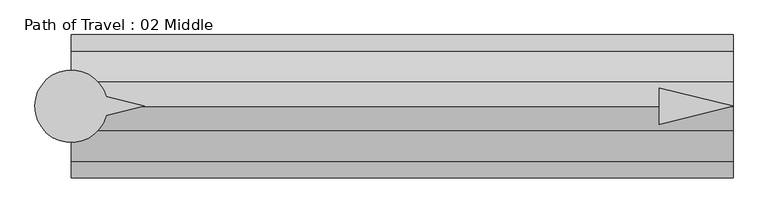
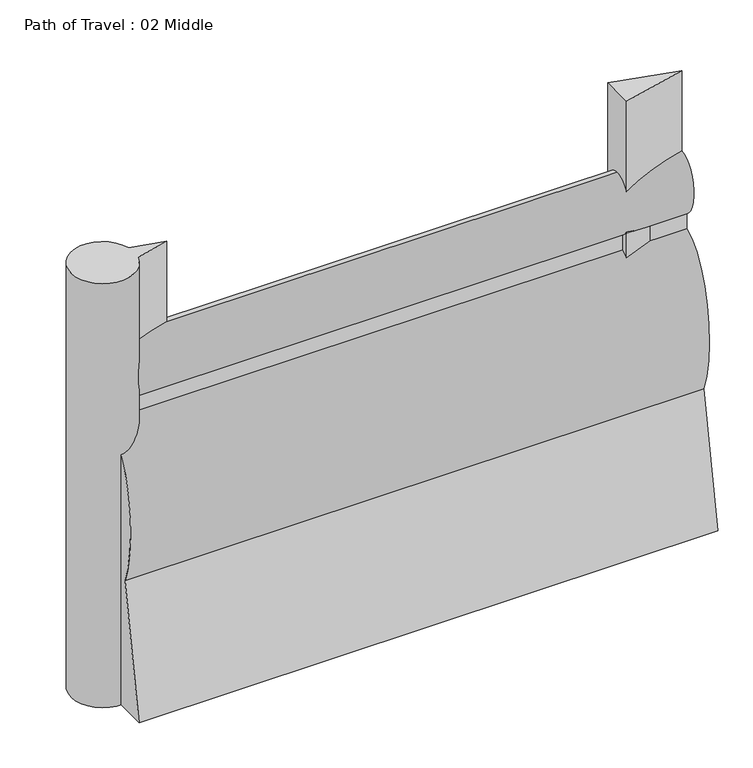
"""IFC4 building model written with IfcOpenShell, lengths in millimetres: proxy geometry, Path of Travel : 02 Middle."""

from ifc_helpers import new_model, si_unit, point, frame, frame_2d, origin, origin_with_axes, place, context, project, spatial, polyline, circle_curve, ellipse_curve, trimmed, segment, composite_curve, outline, extrude, source, transform, mapped, element, save
from ifc_brep_helpers import plane_surface, extruded_surface, advanced_brep


def path_of_travel_02_middle_a2a4b6ed(model_context):
    return source(origin(), model_context, "Body", "SolidModel", [
        advanced_brep(
        [(227.5554837, 0.0, 1727.2), (227.5554837, 42.9018657, 1436.6534209), (227.5554837, 42.9018657, 1363.4763406), (227.5554837, 184.1186263, 643.4144547), (227.5554837, 297.5699544, 0.0), (227.5554837, 145.6574193, 0.0), (227.5554837, 0.0, 584.2), (227.5554837, -145.6574193, 0.0), (227.5554837, -297.5699544, 0.0), (227.5554837, -184.1186263, 643.4144547), (227.5554837, -42.9018657, 1363.4763406), (227.5554837, -42.9018657, 1436.6534209), (2978.9406446, 0.0, 1727.2), (2978.9406446, -42.9018657, 1436.6534209), (2978.9406446, -42.9018657, 1363.4763406), (2978.9406446, -184.1186263, 643.4144547), (2978.9406446, -297.5699544, 0.0), (2978.9406446, -145.6574193, 0.0), (2978.9406446, 0.0, 584.2), (2978.9406446, 145.6574193, 0.0), (2978.9406446, 297.5699544, 0.0), (2978.9406446, 184.1186263, 643.4144547), (2978.9406446, 42.9018657, 1363.4763406), (2978.9406446, 42.9018657, 1436.6534209)],
        [
            (0, 1, ellipse_curve(frame((227.5554837, 0.0, 1574.8), z_axis=(-1.0, 0.0, 0.0), x_axis=(0.0, 0.0, 1.0)), 152.4, 101.6)),
            (1, 2),
            (2, 3, ellipse_curve(frame((227.5554837, 0.0, 914.4), z_axis=(-1.0, 0.0, 0.0), x_axis=(0.0, 0.0, -1.0)), 457.2, 228.6)),
            (3, 4),
            (4, 5),
            (5, 6),
            (6, 7),
            (7, 8),
            (8, 9),
            (9, 10, ellipse_curve(frame((227.5554837, 0.0, 914.4), z_axis=(-1.0, 0.0, 0.0), x_axis=(0.0, 0.0, -1.0)), 457.2, 228.6)),
            (10, 11),
            (11, 0, ellipse_curve(frame((227.5554837, 0.0, 1574.8), z_axis=(-1.0, 0.0, 0.0), x_axis=(0.0, 0.0, 1.0)), 152.4, 101.6)),
            (12, 13, ellipse_curve(frame((2978.9406446, 0.0, 1574.8), z_axis=(1.0, 0.0, 0.0), x_axis=(0.0, 0.0, 1.0)), 152.4, 101.6)),
            (13, 14),
            (14, 15, ellipse_curve(frame((2978.9406446, 0.0, 914.4), z_axis=(1.0, 0.0, 0.0), x_axis=(0.0, 0.0, -1.0)), 457.2, 228.6)),
            (15, 16),
            (16, 17),
            (17, 18),
            (18, 19),
            (19, 20),
            (20, 21),
            (21, 22, ellipse_curve(frame((2978.9406446, 0.0, 914.4), z_axis=(1.0, 0.0, 0.0), x_axis=(0.0, 0.0, -1.0)), 457.2, 228.6)),
            (22, 23),
            (23, 12, ellipse_curve(frame((2978.9406446, 0.0, 1574.8), z_axis=(1.0, 0.0, 0.0), x_axis=(0.0, 0.0, 1.0)), 152.4, 101.6)),
            (0, 12),
            (23, 1),
            (22, 2),
            (21, 3),
            (20, 4),
            (19, 5),
            (18, 6),
            (17, 7),
            (16, 8),
            (15, 9),
            (14, 10),
            (13, 11),
        ],
        [
            plane_surface(frame((227.5554837, 0.0, 0.0), z_axis=(-1.0, 0.0, 0.0), x_axis=(0.0, 0.0, 1.0))),
            plane_surface(frame((2978.9406446, 0.0, 0.0), z_axis=(1.0, 0.0, 0.0), x_axis=(0.0, 0.0, 1.0))),
            extruded_surface(trimmed(ellipse_curve(frame((2978.9406446, 0.0, 1574.8), z_axis=(-1.0, 0.0, 0.0), x_axis=(0.0, 0.0, 1.0)), 152.4, 101.6), [point((2978.9406446, 0.0, 1727.2))], [point((2978.9406446, 42.9018657, 1436.6534209))], True, "CARTESIAN"), (-2751.3851609, 0.0, 0.0), 2751.3851609),
            plane_surface(frame((227.5554837, 42.9018657, 1436.6534209), z_axis=(0.0, 1.0, 0.0), x_axis=(1.0, 0.0, 0.0))),
            extruded_surface(trimmed(ellipse_curve(frame((2978.9406446, 0.0, 914.4), z_axis=(-1.0, 0.0, 0.0), x_axis=(0.0, 0.0, -1.0)), 457.2, 228.6), [point((2978.9406446, 42.9018657, 1363.4763406))], [point((2978.9406446, 184.1186263, 643.4144547))], True, "CARTESIAN"), (-2751.3851609, 0.0, 0.0), 2751.3851609),
            plane_surface(frame((227.5554837, 184.1186263, 643.4144547), z_axis=(0.0, 0.9848077530122078, 0.1736481776669322), x_axis=(1.0, 0.0, 0.0))),
            plane_surface(frame((227.5554837, 297.5699544, 0.0), z_axis=(0.0, 0.0, -1.0), x_axis=(1.0, 0.0, 0.0))),
            plane_surface(frame((227.5554837, 145.6574193, 0.0), z_axis=(0.0, -0.9702957262760199, -0.2419218955995739), x_axis=(1.0, 0.0, 0.0))),
            plane_surface(frame((227.5554837, 0.0, 584.2), z_axis=(0.0, 0.9702957262759961, -0.24192189559966923), x_axis=(1.0, 0.0, 0.0))),
            plane_surface(frame((227.5554837, -145.6574193, 0.0), z_axis=(0.0, 0.0, -1.0), x_axis=(1.0, 0.0, 0.0))),
            plane_surface(frame((227.5554837, -297.5699544, 0.0), z_axis=(0.0, -0.984807753012208, 0.17364817766693066), x_axis=(1.0, 0.0, 0.0))),
            extruded_surface(trimmed(ellipse_curve(frame((2978.9406446, 0.0, 914.4), z_axis=(-1.0, 0.0, 0.0), x_axis=(0.0, 0.0, -1.0)), 457.2, 228.6), [point((2978.9406446, -184.1186263, 643.4144547))], [point((2978.9406446, -42.9018657, 1363.4763406))], True, "CARTESIAN"), (-2751.3851609, 0.0, 0.0), 2751.3851609),
            plane_surface(frame((227.5554837, -42.9018657, 1363.4763406), z_axis=(0.0, -1.0, 0.0), x_axis=(1.0, 0.0, 0.0))),
            extruded_surface(trimmed(ellipse_curve(frame((2978.9406446, 0.0, 1574.8), z_axis=(-1.0, 0.0, 0.0), x_axis=(0.0, 0.0, 1.0)), 152.4, 101.6), [point((2978.9406446, -42.9018657, 1436.6534209))], [point((2978.9406446, 0.0, 1727.2))], True, "CARTESIAN"), (-2751.3851609, 0.0, 0.0), 2751.3851609),
        ],
        [
            (0, [[1, 2, 3, 4, 5, 6, 7, 8, 9, 10, 11, 12]]),
            (1, [[13, 14, 15, 16, 17, 18, 19, 20, 21, 22, 23, 24]]),
            (2, [[-1, 25, -24, 26]]),
            (3, [[-2, -26, -23, 27]]),
            (4, [[-3, -27, -22, 28]]),
            (5, [[-4, -28, -21, 29]]),
            (6, [[-5, -29, -20, 30]]),
            (7, [[-6, -30, -19, 31]]),
            (8, [[-7, -31, -18, 32]]),
            (9, [[-8, -32, -17, 33]]),
            (10, [[-9, -33, -16, 34]]),
            (11, [[-10, -34, -15, 35]]),
            (12, [[-11, -35, -14, 36]]),
            (13, [[-12, -36, -13, -25]]),
        ],
    ),
        extrude(outline(polyline([(2672.9354981, 76.2006338), (2978.9406446, 0.0), (2672.9354981, -76.2006338), (2672.9354981, 76.2006338)])), origin_with_axes(), (0.0, 0.0, 1.0), 2129.5973753),
        extrude(outline(composite_curve([segment(polyline([(372.7837828, 39.4440225), (531.182385, 0.0), (372.7837828, -39.4440225)]), True, "CONTINUOUS"), segment(trimmed(circle_curve(frame_2d((227.2200886, 0.0)), 150.8131956), [point((372.7837828, -39.4440225))], [point((372.7837828, 39.4440225))], False, "CARTESIAN"), True, "CONTINUOUS")], self_intersect=False)), origin_with_axes(), (0.0, 0.0, 1.0), 2129.5973753),
    ])


if __name__ == "__main__":
    model = new_model("IFC4")
    model_context = context("Model", 3, world=origin())
    ifc_project = project(units=[si_unit("LENGTHUNIT", "METRE", prefix="MILLI")], contexts=[model_context])
    site = spatial("IfcSite", under=ifc_project)
    building = spatial("IfcBuilding", under=site)
    placement = place(None, origin())
    path_of_travel_02_middle_shape = path_of_travel_02_middle_a2a4b6ed(model_context)
    element("IfcBuildingElementProxy", 1, Name="Path of Travel : 02 Middle", ObjectType="Path of Travel : 02 Middle", at=placement, inside=building, context=model_context, shape_type="MappedRepresentation", body=[
        mapped(path_of_travel_02_middle_shape, transform((0.0, 0.0, 0.0), x_axis=(1.0, 0.0, 0.0), y_axis=(0.0, 1.0, 0.0), z_axis=(0.0, 0.0, 1.0))),
    ])
    save(model, "model.ifc")

# Revit data of these elements
# Type "Path of Travel : 02 Middle"
#   Path of Egress [instance default] = 4' - 0"
#   built-in parameter 1001306 [instance default] = 4 (stored number, unit not read)
#   Dot at Start = no
#   Arrow in Middle = yes
#   Arrow at End = no
#   Egress Path = none
# Element 1 (IfcBuildingElementProxy, "Path of Travel : 02 Middle")
#   Path of Egress = 9' - 0.32225"
#   built-in parameter 1001306 = 9.02685 (stored number, unit not read)
#   Materials on its faces: "Egress Path Solid", "solid"
# Materials
#   "Egress Path Solid": class "Unassigned", colour RGB 255 128 64, transparency 0.75, Comments = "Rendering appearance not upgraded "
#   "solid": class "Generic", colour RGB 120 120 120, transparency 0, Cost = 0
